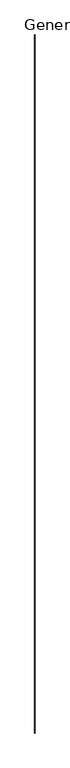
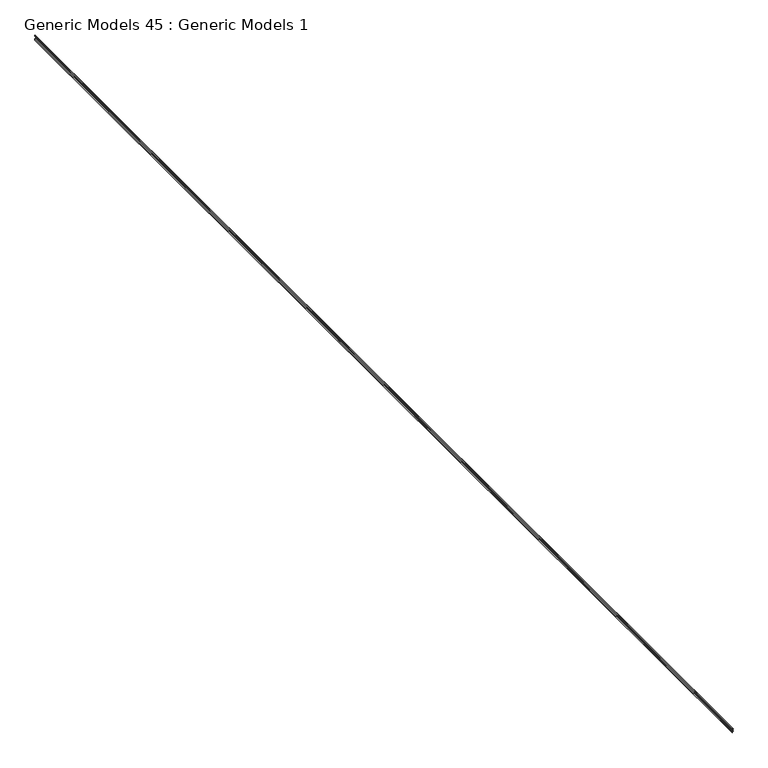
"""IFC4 building model written with IfcOpenShell, lengths in millimetres: proxy geometry, Generic Models 45 : Generic Models 1."""

from ifc_helpers import new_model, si_unit, point, frame, frame_2d, origin, place, context, project, spatial, polyline, circle_curve, trimmed, segment, composite_curve, outline, extrude, source, transform, mapped, element, save


def generic_models_45_generic_models_1_8bb40785(model_context):
    return source(origin(), model_context, "Body", "SweptSolid", [
        extrude(outline(composite_curve([segment(polyline([(266149.1186978, 32152.9864039), (266162.6440287, 32152.9864039), (266162.6440287, 32151.3989039), (266147.8431834, 32151.3989039), (266145.5295602, 32161.8886153)]), True, "CONTINUOUS"), segment(trimmed(circle_curve(frame_2d((266144.7544401, 32161.7176539)), 0.79375), [point((266145.5295602, 32161.8886153))], [point((266144.1628138, 32162.2468205))], True, "CARTESIAN"), True, "CONTINUOUS"), segment(trimmed(circle_curve(frame_2d((266141.2046822, 32164.8926539)), 3.96875), [point((266144.1628138, 32162.2468205))], [point((266141.2046822, 32160.9239039))], False, "CARTESIAN"), True, "CONTINUOUS"), segment(polyline([(266141.2046822, 32160.9239039), (266120.5833752, 32160.9239039)]), True, "CONTINUOUS"), segment(trimmed(circle_curve(frame_2d((266120.5833752, 32164.8926539)), 3.96875), [point((266120.5833752, 32160.9239039))], [point((266117.6252436, 32162.2468205))], False, "CARTESIAN"), True, "CONTINUOUS"), segment(trimmed(circle_curve(frame_2d((266117.0336173, 32161.7176539)), 0.79375), [point((266117.6252436, 32162.2468205))], [point((266116.2584972, 32161.8886153))], True, "CARTESIAN"), True, "CONTINUOUS"), segment(polyline([(266116.2584972, 32161.8886153), (266113.944874, 32151.3989039), (266099.1440287, 32151.3989039), (266099.1440287, 32152.9864039), (266112.6693597, 32152.9864039), (266114.7082569, 32162.2305381)]), True, "CONTINUOUS"), segment(trimmed(circle_curve(frame_2d((266117.0336173, 32161.7176539)), 2.38125), [point((266114.7082569, 32162.2305381))], [point((266118.8084963, 32163.3051539))], False, "CARTESIAN"), True, "CONTINUOUS"), segment(trimmed(circle_curve(frame_2d((266120.5833752, 32164.8926539)), 2.38125), [point((266118.8084963, 32163.3051539))], [point((266120.5833752, 32162.5114039))], True, "CARTESIAN"), True, "CONTINUOUS"), segment(polyline([(266120.5833752, 32162.5114039), (266141.2046822, 32162.5114039)]), True, "CONTINUOUS"), segment(trimmed(circle_curve(frame_2d((266141.2046822, 32164.8926539)), 2.38125), [point((266141.2046822, 32162.5114039))], [point((266142.9795611, 32163.3051539))], True, "CARTESIAN"), True, "CONTINUOUS"), segment(trimmed(circle_curve(frame_2d((266144.7544401, 32161.7176539)), 2.38125), [point((266142.9795611, 32163.3051539))], [point((266147.0798006, 32162.2305381))], False, "CARTESIAN"), True, "CONTINUOUS"), segment(polyline([(266147.0798006, 32162.2305381), (266149.1186978, 32152.9864039)]), True, "CONTINUOUS")], self_intersect=False)), frame((0.0, 25672.1156612, 0.0), z_axis=(0.0, 1.0, 0.0), x_axis=(0.0, 0.0, 1.0)), (0.0, 0.0, 1.0), 15155.545),
    ])


if __name__ == "__main__":
    model = new_model("IFC4")
    model_context = context("Model", 3, world=origin())
    ifc_project = project(units=[si_unit("LENGTHUNIT", "METRE", prefix="MILLI")], contexts=[model_context])
    site = spatial("IfcSite", under=ifc_project)
    building = spatial("IfcBuilding", under=site)
    placement = place(None, origin())
    generic_models_45_generic_models_1_shape = generic_models_45_generic_models_1_8bb40785(model_context)
    element("IfcBuildingElementProxy", 1, Name="Generic Models 45 : Generic Models 1", ObjectType="Generic Models 45 : Generic Models 1", at=placement, inside=building, context=model_context, shape_type="MappedRepresentation", body=[
        mapped(generic_models_45_generic_models_1_shape, transform((0.0, 0.0, 0.0), x_axis=(1.0, 0.0, 0.0), y_axis=(0.0, 1.0, 0.0), z_axis=(0.0, 0.0, 1.0))),
    ])
    save(model, "model.ifc")

# Revit data of these elements
# Element 1 (IfcBuildingElementProxy, "Generic Models 45 : Generic Models 1")
#   Materials on its faces: "1/2\" DEEP GALV. HORTZ. HAT CHANNEL @ XX O.C."
# Materials
#   "1/2\" DEEP GALV. HORTZ. HAT CHANNEL @ XX O.C.": class "Generic", colour RGB 212 212 212, transparency 0, Cost = 0
